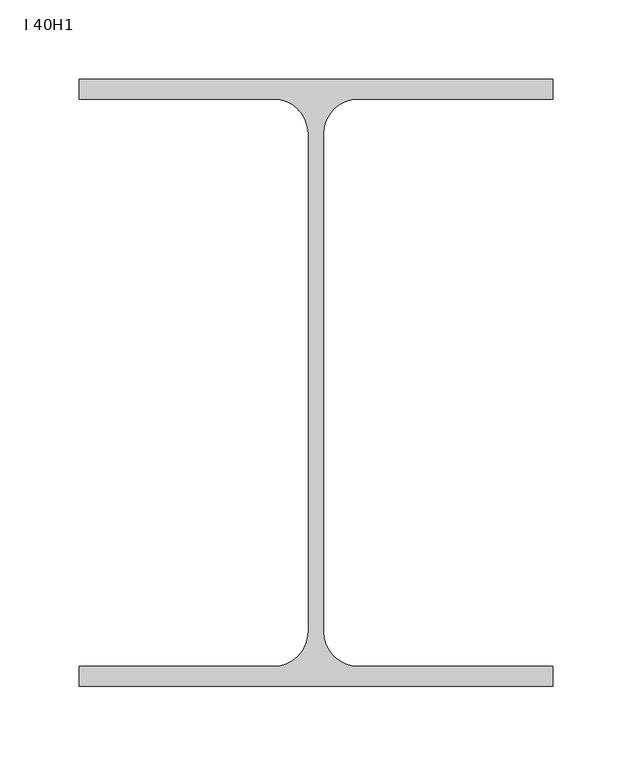
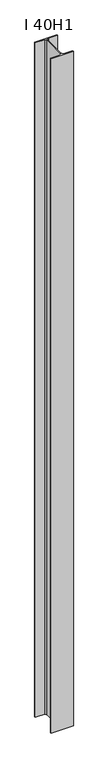
"""IFC4 building model written with IfcOpenShell, lengths in millimetres: column geometry, Двутавровая балка с широкими полками (ASTO20-93)-Колонна : I 40H1."""

from ifc_helpers import new_model, si_unit, point, frame_2d, origin, origin_with_axes, place, context, project, spatial, polyline, circle_curve, trimmed, segment, composite_curve, outline, extrude, source, transform, mapped, element, save


def i_40h1_838be756(model_context):
    return source(origin(), model_context, "Body", "SweptSolid", [
        extrude(outline(composite_curve([segment(polyline([(-149.5, -178.5), (-26.75, -178.5)]), True, "CONTINUOUS"), segment(trimmed(circle_curve(frame_2d((-26.75, -156.5)), 22.0), [point((-26.75, -178.5))], [point((-4.75, -156.5))], True, "CARTESIAN"), True, "CONTINUOUS"), segment(polyline([(-4.75, -156.5), (-4.75, 157.5)]), True, "CONTINUOUS"), segment(trimmed(circle_curve(frame_2d((-26.75, 157.5)), 22.0), [point((-4.75, 157.5))], [point((-26.75, 179.5))], True, "CARTESIAN"), True, "CONTINUOUS"), segment(polyline([(-26.75, 179.5), (-149.5, 179.5), (-149.5, 192.0), (149.5, 192.0), (149.5, 179.5), (26.75, 179.5)]), True, "CONTINUOUS"), segment(trimmed(circle_curve(frame_2d((26.75, 157.5)), 22.0), [point((26.75, 179.5))], [point((4.75, 157.5))], True, "CARTESIAN"), True, "CONTINUOUS"), segment(polyline([(4.75, 157.5), (4.75, -156.5)]), True, "CONTINUOUS"), segment(trimmed(circle_curve(frame_2d((26.75, -156.5)), 22.0), [point((4.75, -156.5))], [point((26.75, -178.5))], True, "CARTESIAN"), True, "CONTINUOUS"), segment(polyline([(26.75, -178.5), (149.5, -178.5), (149.5, -191.0), (-149.5, -191.0), (-149.5, -178.5)]), True, "CONTINUOUS")], self_intersect=False)), origin_with_axes(), (0.0, 0.0, 1.0), 9604.6332616),
    ])


if __name__ == "__main__":
    model = new_model("IFC4")
    model_context = context("Model", 3, world=origin())
    ifc_project = project(units=[si_unit("LENGTHUNIT", "METRE", prefix="MILLI")], contexts=[model_context])
    site = spatial("IfcSite", under=ifc_project)
    building = spatial("IfcBuilding", under=site)
    placement = place(None, origin())
    i_40h1_shape = i_40h1_838be756(model_context)
    element("IfcColumn", 1, ObjectType="Двутавровая балка с широкими полками (ASTO20-93)-Колонна : I 40H1", at=placement, inside=building, context=model_context, shape_type="MappedRepresentation", body=[
        mapped(i_40h1_shape, transform((0.0, 0.0, 0.0), x_axis=(1.0, 0.0, 0.0), y_axis=(0.0, 1.0, 0.0), z_axis=(0.0, 0.0, 1.0))),
    ])
    save(model, "model.ifc")

# Revit data of these elements
# Type "Двутавровая балка с широкими полками (ASTO20-93)-Колонна : I 40H1"
#   ra = 22 mm
#   W = 0.868869
#   Vz = 191.5 mm
#   Vy = 149.5 mm
#   Vpz = 191.5 mm
#   Vpy = 149.5 mm
#   bf = 299 mm
#   d = 383 mm
#   tf = 12.5 mm
#   tw = 9.5 mm
#   A = 0.011291 m²
#   Structural Material [instance default] = Металл - Сталь - 345 МПa
#   Assembly Code = ""
# Element 1 (IfcColumn, "Двутавровая балка с широкими полками (ASTO20-93)-Колонна : I 40H1")
#   Structural Material = C345
#   Materials on its faces: "C345"
# Materials
#   "Металл - Сталь - 345 МПa": class "Металл", colour RGB 247 247 247, transparency 0
#   "C345": class "Не назначено", colour RGB 0 0 0, transparency 0
